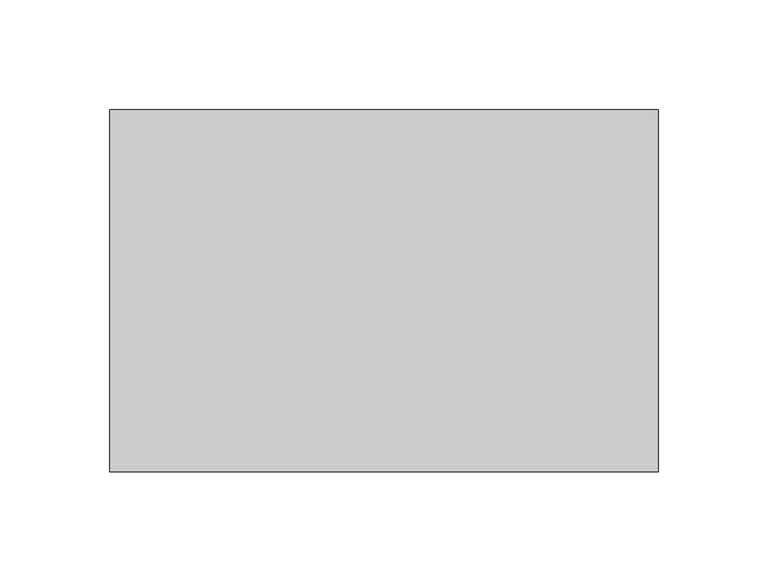
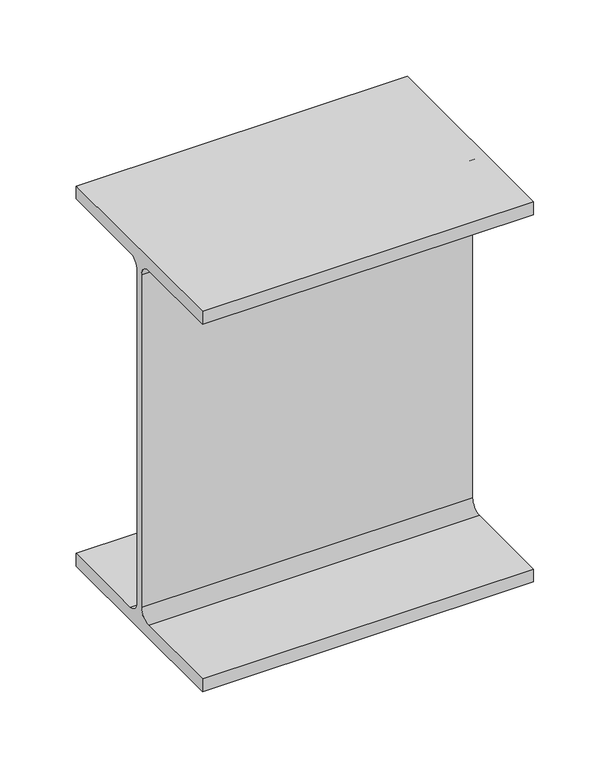
"""IFC4 building model written with IfcOpenShell, lengths in millimetres: beam geometry, Old_Steel Beam_H-KSD3502 : H_SB_ASB_H-300×150x6.5x9."""

from ifc_helpers import new_model, si_unit, point, frame, frame_2d, origin, place, context, project, spatial, polyline, circle_curve, trimmed, segment, composite_curve, outline, extrude, source, transform, mapped, element, save


def beam_e2bb94c7(model_context):
    return source(origin(), model_context, "Body", "SweptSolid", [
        extrude(outline(composite_curve([segment(polyline([(82.5, -141.5), (82.5, -151.7), (-82.5, -151.7), (-82.5, -141.5), (-11.9, -141.5)]), True, "CONTINUOUS"), segment(trimmed(circle_curve(frame_2d((-11.9, -132.6)), 8.9), [point((-11.9, -141.5))], [point((-3.0, -132.6))], True, "CARTESIAN"), True, "CONTINUOUS"), segment(polyline([(-3.0, -132.6), (-3.0, 132.6)]), True, "CONTINUOUS"), segment(trimmed(circle_curve(frame_2d((-11.9, 132.6)), 8.9), [point((-3.0, 132.6))], [point((-11.9, 141.5))], True, "CARTESIAN"), True, "CONTINUOUS"), segment(polyline([(-11.9, 141.5), (-82.5, 141.5), (-82.5, 151.7), (82.5, 151.7), (82.5, 141.5), (11.9, 141.5)]), True, "CONTINUOUS"), segment(trimmed(circle_curve(frame_2d((11.9, 132.6)), 8.9), [point((11.9, 141.5))], [point((3.0, 132.6))], True, "CARTESIAN"), True, "CONTINUOUS"), segment(polyline([(3.0, 132.6), (3.0, -132.6)]), True, "CONTINUOUS"), segment(trimmed(circle_curve(frame_2d((11.9, -132.6)), 8.9), [point((3.0, -132.6))], [point((11.9, -141.5))], True, "CARTESIAN"), True, "CONTINUOUS"), segment(polyline([(11.9, -141.5), (82.5, -141.5)]), True, "CONTINUOUS")], self_intersect=False)), frame((-50.0, 0.0, 0.0), z_axis=(1.0, 0.0, 0.0), x_axis=(0.0, 1.0, 0.0)), (0.0, 0.0, 1.0), 249.9999994),
    ])


if __name__ == "__main__":
    model = new_model("IFC4")
    model_context = context("Model", 3, world=origin())
    ifc_project = project(units=[si_unit("LENGTHUNIT", "METRE", prefix="MILLI")], contexts=[model_context])
    site = spatial("IfcSite", under=ifc_project)
    building = spatial("IfcBuilding", under=site)
    placement = place(None, origin())
    beam_shape = beam_e2bb94c7(model_context)
    element("IfcBeam", 1, ObjectType="Old_Steel Beam_H-KSD3502 : H_SB_ASB_H-300×150x6.5x9", at=placement, inside=building, context=model_context, shape_type="MappedRepresentation", body=[
        mapped(beam_shape, transform((0.0, 0.0, 0.0), x_axis=(1.0, 0.0, 0.0), y_axis=(0.0, 1.0, 0.0), z_axis=(0.0, 0.0, 1.0))),
    ])
    save(model, "model.ifc")

# Revit data of these elements
# Type "Old_Steel Beam_H-KSD3502 : H_SB_ASB_H-300×150x6.5x9"
#   Width = 15.0 cm
#   Web Thickness = 0.65 cm
#   Web Fillet = 1.3 cm
#   Warping Constant = 107174.0 cm⁶
#   Torsional Moment of Inertia = 9.9539 cm⁴
#   Torsional Modulus = 1.0 cm³
#   Section Area = 46.78 cm²
#   Plastic Modulus weak axis = 105.0 cm³
#   Plastic Modulus strong axis = 542.0 cm³
#   Perimeter = 1.17 m²/m
#   Nominal Weight = 36.70 kgf/m
#   Moment of Inertia weak axis = 508.00 cm⁴
#   Moment of Inertia strong axis = 7210.00 cm⁴
#   Height = 30.0 cm
#   Flange Thickness = 0.9 cm
#   Elastic Modulus weak axis = 67.7 cm³
#   Elastic Modulus strong axis = 481.0 cm³
#   Centroid Vertical = 15.0 cm
#   Centroid Horizontal = 7.5 cm
#   Length [instance default] = 1.5240 m
#   Structural Material [instance default] = Steel, 45-345
#   Assembly Code = ""
# Element 1 (IfcBeam, "Old_Steel Beam_H-KSD3502 : H_SB_ASB_H-300×150x6.5x9")
#   Structural Material = none
# Materials
#   "Steel, 45-345": class "Metal", colour RGB 189 187 185, transparency 0, Description = "Steel 345 MPa", Cost = 0
